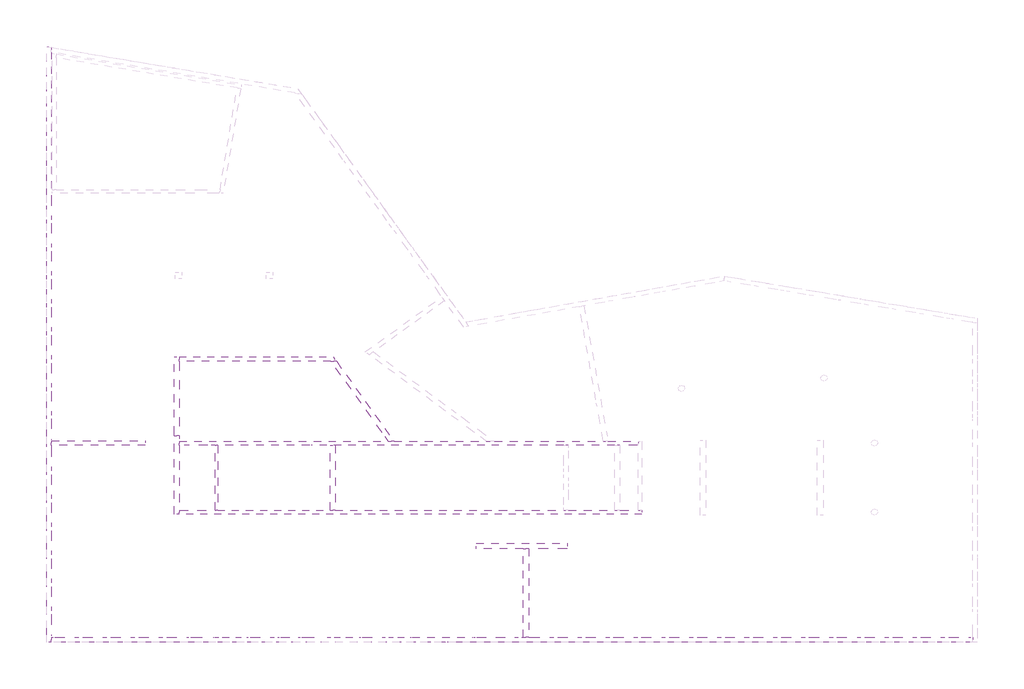
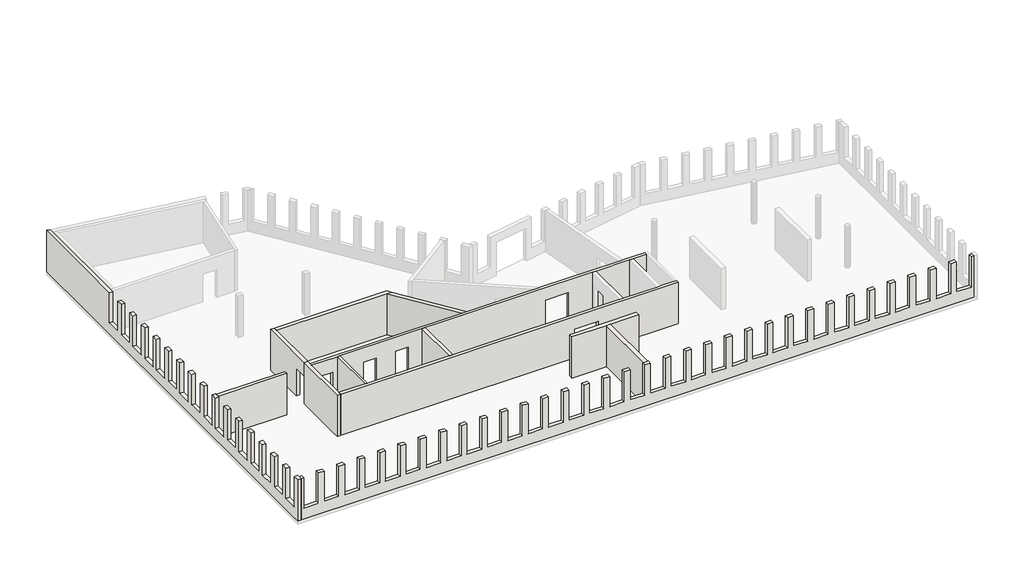
# One storey, part 1 of 2: 13 walls.
# Revit data of these elements (continued)
# Project information (continued)
#   BrowserStrukturXMLData = "<Browserstruktur>\n  <xs:schema id=\"Browserstruktur\" xmlns=\"\" xmlns:xs=\"http://www.w3.org/2001/XMLSchema\" xmlns:msdata=\"urn:schemas-microsoft-com:xml-msdata\">\n    <xs:element name=\"Browserstruktur\" msdata:IsDataSet=\"true\" msdata:MainDataTable=\"ViewTemplates\" msdata:UseCurrentLocale=\"true\">\n      <xs:complexType>\n        <xs:choice minOccurs=\"0\" maxOccurs=\"unbounded\">\n          <xs:element name=\"ViewTemplates\">\n            <xs:complexType>\n              <xs:sequence>\n                <xs:element name=\"Erstellen\" type=\"xs:boolean\" minOccurs=\"0\" />\n                <xs:element name=\"Ansichtsvorlage\" type=\"xs:string\" />\n                <xs:element name=\"_x0031__Fachbereich\" type=\"xs:string\" minOccurs=\"0\" />\n                <xs:element name=\"_x0032__Ansichtstyp\" type=\"xs:string\" minOccurs=\"0\" />\n                <xs:element name=\"_x0033__Ansichtsgruppe\" type=\"xs:string\" minOccurs=\"0\" />\n                <xs:element name=\"Typ\" type=\"xs:string\" minOccurs=\"0\" />\n                <xs:element name=\"Klasse\" type=\"xs:string\" minOccurs=\"0\" />\n                <xs:element name=\"Bedingung\" type=\"xs:string\" minOccurs=\"0\" />\n                <xs:element name=\"Ebenenbezug\" type=\"xs:int\" minOccurs=\"0\" />\n                <xs:element name=\"Ansichtsrichtung\" type=\"xs:string\" minOccurs=\"0\" />\n                <xs:element name=\"Ansichtsname\" type=\"xs:string\" minOccurs=\"0\" />\n              </xs:sequence>\n            </xs:complexType>\n          </xs:element>\n        </xs:choice>\n      </xs:complexType>\n      <xs:unique name=\"Constraint1\" msdata:PrimaryKey=\"true\">\n        <xs:selector xpath=\".//ViewTemplates\" />\n        <xs:field xpath=\"Ansichtsvorlage\" />\n      </xs:unique>\n    </xs:element>\n  </xs:schema>\n  <ViewTemplates>\n    <Erstellen>false</Erstellen>\n    <Ansichtsvorlage>010</Ansichtsvorlage>\n    <_x0031__Fachbereich>00_INTERN</_x0031__Fachbereich>\n    <_x0032__Ansichtstyp>010_CAD_UNTERLAGE</_x0032__Ansichtstyp>\n    <_x0033__Ansichtsgruppe>010_UNTERLAGE_CAD_GESAMT</_x0033__Ansichtsgruppe>\n    <Typ>FloorPlan</Typ>\n    <Klasse>ViewPlan</Klasse>\n    <Bedingung>einmalig</Bedingung>\n    <Ansichtsrichtung>&lt;Ignorieren&gt;</Ansichtsrichtung>\n    <Ansichtsname>[Geschoss_Name]_[Ansichtsgruppe_Name]_[Ebenen_Kommentar]</Ansichtsname>\n  </ViewTemplates>\n  <ViewTemplates>\n    <Erstellen>false</Erstellen>\n    <Ansichtsvorlage>011</Ansichtsvorlage>\n    <_x0031__Fachbereich>00_INTERN</_x0031__Fachbereich>\n    <_x0032__Ansichtstyp>010_CAD_UNTERLAGE</_x0032__Ansichtstyp>\n    <_x0033__Ansichtsgruppe>011_LAGEPLAN</_x0033__Ansichtsgruppe>\n    <Typ>FloorPlan</Typ>\n    <Klasse>ViewPlan</Klasse>\n    <Bedingung>einmalig</Bedingung>\n    <Ansichtsrichtung>&lt;Ignorieren&gt;</Ansichtsrichtung>\n    <Ansichtsname>[Geschoss_Name]_[Ansichtsgruppe_Name]_[Ebenen_Kommentar]</Ansichtsname>\n  </ViewTemplates>\n  <ViewTemplates>\n    <Erstellen>false</Erstellen>\n    <Ansichtsvorlage>025</Ansichtsvorlage>\n    <_x0031__Fachbereich>00_INTERN</_x0031__Fachbereich>\n    <_x0032__Ansichtstyp>010_CAD_UNTERLAGE</_x0032__Ansichtstyp>\n    <_x0033__Ansichtsgruppe>025_ACHSEN</_x0033__Ansichtsgruppe>\n    <Typ>FloorPlan</Typ>\n    <Klasse>ViewPlan</Klasse>\n    <Bedingung>einmalig</Bedingung>\n    <Ansichtsrichtung>&lt;Ignorieren&gt;</Ansichtsrichtung>\n    <Ansichtsname>[Geschoss_Name]_[Ansichtsgruppe_Name]_[Ebenen_Kommentar]</Ansichtsname>\n  </ViewTemplates>\n  <ViewTemplates>\n    <Erstellen>false</Erstellen>\n    <Ansichtsvorlage>030</Ansichtsvorlage>\n    <_x0031__Fachbereich>00_INTERN</_x0031__Fachbereich>\n    <_x0032__Ansichtstyp>010_CAD_UNTERLAGE</_x0032__Ansichtstyp>\n    <_x0033__Ansichtsgruppe>030_ENTWURF_ARCHITEKT</_x0033__Ansichtsgruppe>\n    <Typ>FloorPlan</Typ>\n    <Klasse>ViewPlan</Klasse>\n    <Bedingung>einmalig</Bedingung>\n    <Ebenenbezug>100</Ebenenbezug>\n    <Ansichtsrichtung>&lt;Ignorieren&gt;</Ansichtsrichtung>\n    <Ansichtsname>[Geschoss_Name]_[Ansichtsgruppe_Name]_[Ebenen_Kommentar]</Ansichtsname>\n  </ViewTemplates>\n  <ViewTemplates>\n    <Erstellen>false</Erstellen>\n    <Ansichtsvorlage>060</Ansichtsvorlage>\n    <_x0031__Fachbereich>00_INTERN</_x0031__Fachbereich>\n    <_x0032__Ansichtstyp>060_BILD_UNTERLAGE</_x0032__Ansichtstyp>\n    <_x0033__Ansichtsgruppe>060_UNTERLAGE_BITMAP</_x0033__Ansichtsgruppe>\n    <Typ>FloorPlan</Typ>\n    <Klasse>ViewPlan</Klasse>\n    <Bedingung>einmalig</Bedingung>\n    <Ansichtsrichtung>&lt;Ignorieren&gt;</Ansichtsrichtung>\n    <Ansichtsname>[Geschoss_Name]_[Ansichtsgruppe_Name]_[Ebenen_Kommentar]</Ansichtsname>\n  </ViewTemplates>\n  <ViewTemplates>\n    <Erstellen>false</Erstellen>\n    <Ansichtsvorlage>070</Ansichtsvorlage>\n    <_x0031__Fachbereich>00_INTERN</_x0031__Fachbereich>\n    <_x0032__Ansichtstyp>070_CAD_UEBERLAGE</_x0032__Ansichtstyp>\n    <_x0033__Ansichtsgruppe>070_UEBERLAGE_CAD</_x0033__Ansichtsgruppe>\n    <Typ>FloorPlan</Typ>\n    <Klasse>ViewPlan</Klasse>\n    <Bedingung>einmalig</Bedingung>\n    <Ansichtsrichtung>&lt;Ignorieren&gt;</Ansichtsrichtung>\n    <Ansichtsname>[Geschoss_Name]_[Ansichtsgruppe_Name]_[Ebenen_Kommentar]</Ansichtsname>\n  </ViewTemplates>\n  <ViewTemplates>\n    <Erstellen>false</Erstellen>\n    <Ansichtsvorlage>080</Ansichtsvorlage>\n    <_x0031__Fachbereich>00_INTERN</_x0031__Fachbereich>\n    <_x0032__Ansichtstyp>080_BILD_UEBERLAGE</_x0032__Ansichtstyp>\n    <_x0033__Ansichtsgruppe>080_UEBERLAGE_BITMAP</_x0033__Ansichtsgruppe>\n    <Typ>FloorPlan</Typ>\n    <Klasse>ViewPlan</Klasse>\n    <Bedingung>einmalig</Bedingung>\n    <Ansichtsrichtung>&lt;Ignorieren&gt;</Ansichtsrichtung>\n    <Ansichtsname>[Geschoss_Name]_[Ansichtsgruppe_Name]_[Ebenen_Kommentar]</Ansichtsname>\n  </ViewTemplates>\n  <ViewTemplates>\n    <Erstellen>false</Erstellen>\n    <Ansichtsvorlage>K_5_CC</Ansichtsvorlage>\n    <_x0031__Fachbereich>K_KONSTRUKTION</_x0031__Fachbereich>\n    <_x0032__Ansichtstyp>5_INGENIEUR / ROHBAU</_x0032__Ansichtstyp>\n    <_x0033__Ansichtsgruppe>5_CC_WÄNDE/STÜTZEN</_x0033__Ansichtsgruppe>\n    <Typ>FloorPlan</Typ>\n    <Klasse>ViewPlan</Klasse>\n    <Bedingung>Für jedes Geschoß</Bedingung>\n    <Ebenenbezug>-2</Ebenenbezug>\n    <Ansichtsrichtung>&lt;Ignorieren&gt;</Ansichtsrichtung>\n    <Ansichtsname>[Geschoss_Name]_[Ansichtsgruppe_Name]_[Ebenen_Kommentar]</Ansichtsname>\n  </ViewTemplates>\n  <ViewTemplates>\n    <Erstellen>false</Erstellen>\n    <Ansichtsvorlage>K_5_AA</Ansichtsvorlage>\n    <_x0031__Fachbereich>K_KONSTRUKTION</_x0031__Fachbereich>\n    <_x0032__Ansichtstyp>5_INGENIEUR / ROHBAU</_x0032__Ansichtstyp>\n    <_x0033__Ansichtsgruppe>5_AA_FUNDAMENTE</_x0033__Ansichtsgruppe>\n    <Typ>FloorPlan</Typ>\n    <Klasse>ViewPlan</Klasse>\n    <Bedingung>Für jedes Geschoß</Bedingung>\n    <Ebenenbezug>1000</Ebenenbezug>\n    <Ansichtsrichtung>&lt;Ignorieren&gt;</Ansichtsrichtung>\n    <Ansichtsname>[Geschoss_Name]_[Ansichtsgruppe_Name]_[Ebenen_Kommentar]</Ansichtsname>\n  </ViewTemplates>\n  <ViewTemplates>\n    <Erstellen>false</Erstellen>\n    <Ansichtsvorlage>K_5_BB</Ansichtsvorlage>\n    <_x0031__Fachbereich>K_KONSTRUKTION</_x0031__Fachbereich>\n    <_x0032__Ansichtstyp>5_INGENIEUR / ROHBAU</_x0032__Ansichtstyp>\n    <_x0033__Ansichtsgruppe>5_BB_BODENPLATTE</_x0033__Ansichtsgruppe>\n    <Typ>FloorPlan</Typ>\n    <Klasse>ViewPlan</Klasse>\n    <Bedingung>Für jedes Geschoß</Bedingung>\n    <Ebenenbezug>2</Ebenenbezug>\n    <Ansichtsrichtung>&lt;Ignorieren&gt;</Ansichtsrichtung>\n    <Ansichtsname>[Geschoss_Name]_[Ansichtsgruppe_Name]_[Ebenen_Kommentar]</Ansichtsname>\n  </ViewTemplates>\n  <ViewTemplates>\n    <Erstellen>false</Erstellen>\n    <Ansichtsvorlage>K_5_EE</Ansichtsvorlage>\n    <_x0031__Fachbereich>K_KONSTRUKTION</_x0031__Fachbereich>\n    <_x0032__Ansichtstyp>5_INGENIEUR / ROHBAU</_x0032__Ansichtstyp>\n    <_x0033__Ansichtsgruppe>5_EE_GESCHOSSDECKEN</_x0033__Ansichtsgruppe>\n    <Typ>FloorPlan</Typ>\n    <Klasse>ViewPlan</Klasse>\n    <Bedingung>Für jedes Geschoß</Bedingung>\n    <Ebenenbezug>2</Ebenenbezug>\n    <Ansichtsrichtung>&lt;Ignorieren&gt;</Ansichtsrichtung>\n    <Ansichtsname>[Geschoss_Name]_[Ansichtsgruppe_Name]_[Ebenen_Kommentar]</Ansichtsname>\n  </ViewTemplates>\n  <ViewTemplates>\n    <Erstellen>false</Erstellen>\n    <Ansichtsvorlage>K_6b_AA</Ansichtsvorlage>\n    <_x0031__Fachbereich>K_KONSTRUKTION</_x0031__Fachbereich>\n    <_x0032__Ansichtstyp>6b_FASSADE</_x0032__Ansichtstyp>\n    <_x0033__Ansichtsgruppe>6b_AA_FENSTER_UND_GLASFASSADE</_x0033__Ansichtsgruppe>\n    <Typ>FloorPlan</Typ>\n    <Klasse>ViewPlan</Klasse>\n    <Bedingung>Für jedes Geschoß</Bedingung>\n    <Ebenenbezug>-2</Ebenenbezug>\n    <Ansichtsrichtung>&lt;Ignorieren&gt;</Ansichtsrichtung>\n    <Ansichtsname>[Geschoss_Name]_[Ansichtsgruppe_Name]_[Ebenen_Kommentar]</Ansichtsname>\n  </ViewTemplates>\n  <ViewTemplates>\n    <Erstellen>false</Erstellen>\n    <Ansichtsvorlage>K_6b_DD</Ansichtsvorlage>\n    <_x0031__Fachbereich>K_KONSTRUKTION</_x0031__Fachbereich>\n    <_x0032__Ansichtstyp>6b_FASSADE</_x0032__Ansichtstyp>\n    <_x0033__Ansichtsgruppe>6b_DD_AUßENPUTZ_WDVS</_x0033__Ansichtsgruppe>\n    <Typ>FloorPlan</Typ>\n    <Klasse>ViewPlan</Klasse>\n    <Bedingung>Für jedes Geschoß</Bedingung>\n    <Ebenenbezug>-2</Ebenenbezug>\n    <Ansichtsrichtung>&lt;Ignorieren&gt;</Ansichtsrichtung>\n    <Ansichtsname>[Geschoss_Name]_[Ansichtsgruppe_Name]_[Ebenen_Kommentar]</Ansichtsname>\n  </ViewTemplates>\n  <ViewTemplates>\n    <Erstellen>false</Erstellen>\n    <Ansichtsvorlage>K_5_S1_AA</Ansichtsvorlage>\n    <_x0031__Fachbereich>K_KONSTRUKTION</_x0031__Fachbereich>\n    <_x0032__Ansichtstyp>5_S1_STATIK</_x0032__Ansichtstyp>\n    <_x0033__Ansichtsgruppe>5_S1_AA_GRUNDRISSE</_x0033__Ansichtsgruppe>\n    <Typ>FloorPlan</Typ>\n    <Klasse>ViewPlan</Klasse>\n    <Bedingung>Für jedes Geschoß</Bedingung>\n    <Ebenenbezug>-2</Ebenenbezug>\n    <Ansichtsrichtung>&lt;Ignorieren&gt;</Ansichtsrichtung>\n    <Ansichtsname>[Geschoss_Name]_[Ansichtsgruppe_Name]_[Ebenen_Kommentar]</Ansichtsname>\n  </ViewTemplates>\n  <ViewTemplates>\n    <Erstellen>false</Erstellen>\n    <Ansichtsvorlage>K_5_S2_AA</Ansichtsvorlage>\n    <_x0031__Fachbereich>K_KONSTRUKTION</_x0031__Fachbereich>\n    <_x0032__Ansichtstyp>5_S2_BEWEHRUNG</_x0032__Ansichtstyp>\n    <_x0033__Ansichtsgruppe>5_S2_AA_GRUNDRISSE</_x0033__Ansichtsgruppe>\n    <Typ>FloorPlan</Typ>\n    <Klasse>ViewPlan</Klasse>\n    <Bedingung>Für jedes Geschoß</Bedingung>\n    <Ebenenbezug>-2</Ebenenbezug>\n    <Ansichtsrichtung>&lt;Ignorieren&gt;</Ansichtsrichtung>\n    <Ansichtsname>[Geschoss_Name]_[Ansichtsgruppe_Name]_[Ebenen_Kommentar]</Ansichtsname>\n  </ViewTemplates>\n  <ViewTemplates>\n    <Erstellen>false</Erstellen>\n    <Ansichtsvorlage>K_5_DD</Ansichtsvorlage>\n    <_x0031__Fachbereich>K_KONSTRUKTION</_x0031__Fachbereich>\n    <_x0032__Ansichtstyp>5_INGENIEUR / ROHBAU</_x0032__Ansichtstyp>\n    <_x0033__Ansichtsgruppe>5_DD_TRÄGER</_x0033__Ansichtsgruppe>\n    <Typ>FloorPlan</Typ>\n    <Klasse>ViewPlan</Klasse>\n    <Bedingung>Für jedes Geschoß</Bedingung>\n    <Ebenenbezug>1</Ebenenbezug>\n    <Ansichtsrichtung>&lt;Ignorieren&gt;</Ansichtsrichtung>\n    <Ansichtsname>[Geschoss_Name]_[Ansichtsgruppe_Name]_[Ebenen_Kommentar]</Ansichtsname>\n  </ViewTemplates>\n  <ViewTemplates>\n    <Erstellen>false</Erstellen>\n    <Ansichtsvorlage>K_5_S1_BB</Ansichtsvorlage>\n    <_x0031__Fachbereich>K_KONSTRUKTION</_x0031__Fachbereich>\n    <_x0032__Ansichtstyp>5_S1_STATIK</_x0032__Ansichtstyp>\n    <_x0033__Ansichtsgruppe>5_S1_BB_DECKENSPIEGEL</_x0033__Ansichtsgruppe>\n    <Typ>FloorPlan</Typ>\n    <Klasse>ViewPlan</Klasse>\n    <Bedingung>Für jedes Geschoß</Bedingung>\n    <Ebenenbezug>2</Ebenenbezug>\n    <Ansichtsrichtung>&lt;Ignorieren&gt;</Ansichtsrichtung>\n    <Ansichtsname>[Geschoss_Name]_[Ansichtsgruppe_Name]_[Ebenen_Kommentar]</Ansichtsname>\n  </ViewTemplates>\n  <ViewTemplates>\n    <Erstellen>false</Erstellen>\n    <Ansichtsvor
#     lage>K_5_S2_BB</Ansichtsvorlage>\n    <_x0031__Fachbereich>K_KONSTRUKTION</_x0031__Fachbereich>\n    <_x0032__Ansichtstyp>5_S2_BEWEHRUNG</_x0032__Ansichtstyp>\n    <_x0033__Ansichtsgruppe>5_S2_BB_DECKENSPIEGEL</_x0033__Ansichtsgruppe>\n    <Typ>FloorPlan</Typ>\n    <Klasse>ViewPlan</Klasse>\n    <Bedingung>Für jedes Geschoß</Bedingung>\n    <Ebenenbezug>2</Ebenenbezug>\n    <Ansichtsrichtung>&lt;Ignorieren&gt;</Ansichtsrichtung>\n    <Ansichtsname>[Geschoss_Name]_[Ansichtsgruppe_Name]_[Ebenen_Kommentar]</Ansichtsname>\n  </ViewTemplates>\n  <ViewTemplates>\n    <Erstellen>false</Erstellen>\n    <Ansichtsvorlage>K_6b_BB</Ansichtsvorlage>\n    <_x0031__Fachbereich>K_KONSTRUKTION</_x0031__Fachbereich>\n    <_x0032__Ansichtstyp>6b_FASSADE</_x0032__Ansichtstyp>\n    <_x0033__Ansichtsgruppe>6b_BB_FASSADENBEKLEIDUNG</_x0033__Ansichtsgruppe>\n    <Typ>FloorPlan</Typ>\n    <Klasse>ViewPlan</Klasse>\n    <Bedingung>Für jedes Geschoß</Bedingung>\n    <Ebenenbezug>2</Ebenenbezug>\n    <Ansichtsrichtung>&lt;Ignorieren&gt;</Ansichtsrichtung>\n    <Ansichtsname>[Geschoss_Name]_[Ansichtsgruppe_Name]_[Ebenen_Kommentar]</Ansichtsname>\n  </ViewTemplates>\n  <ViewTemplates>\n    <Erstellen>false</Erstellen>\n    <Ansichtsvorlage>K_6b_CC</Ansichtsvorlage>\n    <_x0031__Fachbereich>K_KONSTRUKTION</_x0031__Fachbereich>\n    <_x0032__Ansichtstyp>6b_FASSADE</_x0032__Ansichtstyp>\n    <_x0033__Ansichtsgruppe>6b_CC_SONNENSCHUTZ_BLENDSCHUTZ</_x0033__Ansichtsgruppe>\n    <Typ>FloorPlan</Typ>\n    <Klasse>ViewPlan</Klasse>\n    <Bedingung>Für jedes Geschoß</Bedingung>\n    <Ebenenbezug>2</Ebenenbezug>\n    <Ansichtsrichtung>&lt;Ignorieren&gt;</Ansichtsrichtung>\n    <Ansichtsname>[Geschoss_Name]_[Ansichtsgruppe_Name]_[Ebenen_Kommentar]</Ansichtsname>\n  </ViewTemplates>\n  <ViewTemplates>\n    <Erstellen>false</Erstellen>\n    <Ansichtsvorlage>K_6c_AA</Ansichtsvorlage>\n    <_x0031__Fachbereich>K_KONSTRUKTION</_x0031__Fachbereich>\n    <_x0032__Ansichtstyp>6c_AUSBAU</_x0032__Ansichtstyp>\n    <_x0033__Ansichtsgruppe>6c_AA_WÄNDE_ALLGEMEIN</_x0033__Ansichtsgruppe>\n    <Typ>FloorPlan</Typ>\n    <Klasse>ViewPlan</Klasse>\n    <Bedingung>Für jedes Geschoß</Bedingung>\n    <Ebenenbezug>-2</Ebenenbezug>\n    <Ansichtsrichtung>&lt;Ignorieren&gt;</Ansichtsrichtung>\n    <Ansichtsname>[Geschoss_Name]_[Ansichtsgruppe_Name]_[Ebenen_Kommentar]</Ansichtsname>\n  </ViewTemplates>\n  <ViewTemplates>\n    <Erstellen>false</Erstellen>\n    <Ansichtsvorlage>K_6c_AC</Ansichtsvorlage>\n    <_x0031__Fachbereich>K_KONSTRUKTION</_x0031__Fachbereich>\n    <_x0032__Ansichtstyp>6c_AUSBAU</_x0032__Ansichtstyp>\n    <_x0033__Ansichtsgruppe>6c_AC_SYSTEMTRENNWÄNDE</_x0033__Ansichtsgruppe>\n    <Typ>FloorPlan</Typ>\n    <Klasse>ViewPlan</Klasse>\n    <Bedingung>Für jedes Geschoß</Bedingung>\n    <Ebenenbezug>3</Ebenenbezug>\n    <Ansichtsrichtung>&lt;Ignorieren&gt;</Ansichtsrichtung>\n    <Ansichtsname>[Geschoss_Name]_[Ansichtsgruppe_Name]_[Ebenen_Kommentar]</Ansichtsname>\n  </ViewTemplates>\n  <ViewTemplates>\n    <Erstellen>false</Erstellen>\n    <Ansichtsvorlage>K_6c_BX</Ansichtsvorlage>\n    <_x0031__Fachbereich>K_KONSTRUKTION</_x0031__Fachbereich>\n    <_x0032__Ansichtstyp>6c_AUSBAU</_x0032__Ansichtstyp>\n    <_x0033__Ansichtsgruppe>6c_BX_RÄUME (RAUMBEZEICHNUNGEN)</_x0033__Ansichtsgruppe>\n    <Typ>FloorPlan</Typ>\n    <Klasse>ViewPlan</Klasse>\n    <Bedingung>Für jedes Geschoß</Bedingung>\n    <Ebenenbezug>3</Ebenenbezug>\n    <Ansichtsrichtung>&lt;Ignorieren&gt;</Ansichtsrichtung>\n    <Ansichtsname>[Geschoss_Name]_[Ansichtsgruppe_Name]_[Ebenen_Kommentar]</Ansichtsname>\n  </ViewTemplates>\n  <ViewTemplates>\n    <Erstellen>false</Erstellen>\n    <Ansichtsvorlage>K_6c_BY</Ansichtsvorlage>\n    <_x0031__Fachbereich>K_KONSTRUKTION</_x0031__Fachbereich>\n    <_x0032__Ansichtstyp>6c_AUSBAU</_x0032__Ansichtstyp>\n    <_x0033__Ansichtsgruppe>6c_BY_RÄUME (NUTZFLÄCHEN NACH DIN 277)</_x0033__Ansichtsgruppe>\n    <Typ>FloorPlan</Typ>\n    <Klasse>ViewPlan</Klasse>\n    <Bedingung>Für jedes Geschoß</Bedingung>\n    <Ebenenbezug>3</Ebenenbezug>\n    <Ansichtsrichtung>&lt;Ignorieren&gt;</Ansichtsrichtung>\n    <Ansichtsname>[Geschoss_Name]_[Ansichtsgruppe_Name]_[Ebenen_Kommentar]</Ansichtsname>\n  </ViewTemplates>\n  <ViewTemplates>\n    <Erstellen>false</Erstellen>\n    <Ansichtsvorlage>K_6c_CA</Ansichtsvorlage>\n    <_x0031__Fachbereich>K_KONSTRUKTION</_x0031__Fachbereich>\n    <_x0032__Ansichtstyp>6c_AUSBAU</_x0032__Ansichtstyp>\n    <_x0033__Ansichtsgruppe>6c_CA_TÜREN_ALLGEMEIN</_x0033__Ansichtsgruppe>\n    <Typ>FloorPlan</Typ>\n    <Klasse>ViewPlan</Klasse>\n    <Bedingung>Für jedes Geschoß</Bedingung>\n    <Ebenenbezug>-2</Ebenenbezug>\n    <Ansichtsrichtung>&lt;Ignorieren&gt;</Ansichtsrichtung>\n    <Ansichtsname>[Geschoss_Name]_[Ansichtsgruppe_Name]_[Ebenen_Kommentar]</Ansichtsname>\n  </ViewTemplates>\n  <ViewTemplates>\n    <Erstellen>false</Erstellen>\n    <Ansichtsvorlage>K_6c_CB</Ansichtsvorlage>\n    <_x0031__Fachbereich>K_KONSTRUKTION</_x0031__Fachbereich>\n    <_x0032__Ansichtstyp>6c_AUSBAU</_x0032__Ansichtstyp>\n    <_x0033__Ansichtsgruppe>6c_CB_HOLZTÜREN (TYPEN)</_x0033__Ansichtsgruppe>\n    <Typ>FloorPlan</Typ>\n    <Klasse>ViewPlan</Klasse>\n    <Bedingung>Für jedes Geschoß</Bedingung>\n    <Ebenenbezug>-2</Ebenenbezug>\n    <Ansichtsrichtung>&lt;Ignorieren&gt;</Ansichtsrichtung>\n    <Ansichtsname>[Geschoss_Name]_[Ansichtsgruppe_Name]_[Ebenen_Kommentar]</Ansichtsname>\n  </ViewTemplates>\n  <ViewTemplates>\n    <Erstellen>false</Erstellen>\n    <Ansichtsvorlage>K_6c_CC</Ansichtsvorlage>\n    <_x0031__Fachbereich>K_KONSTRUKTION</_x0031__Fachbereich>\n    <_x0032__Ansichtstyp>6c_AUSBAU</_x0032__Ansichtstyp>\n    <_x0033__Ansichtsgruppe>6c_CC_BLECHTÜREN (TYPEN)</_x0033__Ansichtsgruppe>\n    <Typ>FloorPlan</Typ>\n    <Klasse>ViewPlan</Klasse>\n    <Bedingung>Für jedes Geschoß</Bedingung>\n    <Ebenenbezug>-2</Ebenenbezug>\n    <Ansichtsrichtung>&lt;Ignorieren&gt;</Ansichtsrichtung>\n    <Ansichtsname>[Geschoss_Name]_[Ansichtsgruppe_Name]_[Ebenen_Kommentar]</Ansichtsname>\n  </ViewTemplates>\n  <ViewTemplates>\n    <Erstellen>false</Erstellen>\n    <Ansichtsvorlage>K_6c_CD</Ansichtsvorlage>\n    <_x0031__Fachbereich>K_KONSTRUKTION</_x0031__Fachbereich>\n    <_x0032__Ansichtstyp>6c_AUSBAU</_x0032__Ansichtstyp>\n    <_x0033__Ansichtsgruppe>6c_CD_ROHRRAHMENTÜREN (TYPEN)</_x0033__Ansichtsgruppe>\n    <Typ>FloorPlan</Typ>\n    <Klasse>ViewPlan</Klasse>\n    <Bedingung>Für jedes Geschoß</Bedingung>\n    <Ebenenbezug>-2</Ebenenbezug>\n    <Ansichtsrichtung>&lt;Ignorieren&gt;</Ansichtsrichtung>\n    <Ansichtsname>[Geschoss_Name]_[Ansichtsgruppe_Name]_[Ebenen_Kommentar]</Ansichtsname>\n  </ViewTemplates>\n  <ViewTemplates>\n    <Erstellen>false</Erstellen>\n    <Ansichtsvorlage>K_6c_CE</Ansichtsvorlage>\n    <_x0031__Fachbereich>K_KONSTRUKTION</_x0031__Fachbereich>\n    <_x0032__Ansichtstyp>6c_AUSBAU</_x0032__Ansichtstyp>\n    <_x0033__Ansichtsgruppe>6c_CE_SPEZIALTÜREN/TORE</_x0033__Ansichtsgruppe>\n    <Typ>FloorPlan</Typ>\n    <Klasse>ViewPlan</Klasse>\n    <Bedingung>Für jedes Geschoß</Bedingung>\n    <Ebenenbezug>-2</Ebenenbezug>\n    <Ansichtsrichtung>&lt;Ignorieren&gt;</Ansichtsrichtung>\n    <Ansichtsname>[Geschoss_Name]_[Ansichtsgruppe_Name]_[Ebenen_Kommentar]</Ansichtsname>\n  </ViewTemplates>\n  <ViewTemplates>\n    <Erstellen>false</Erstellen>\n    <Ansichtsvorlage>K_6c_DA</Ansichtsvorlage>\n    <_x0031__Fachbereich>K_KONSTRUKTION</_x0031__Fachbereich>\n    <_x0032__Ansichtstyp>6c_AUSBAU</_x0032__Ansichtstyp>\n    <_x0033__Ansichtsgruppe>6c_DA_BODENKONSTRUKTION (TYPEN)</_x0033__Ansichtsgruppe>\n    <Typ>FloorPlan</Typ>\n    <Klasse>ViewPlan</Klasse>\n    <Bedingung>Für jedes Geschoß</Bedingung>\n    <Ebenenbezug>3</Ebenenbezug>\n    <Ansichtsrichtung>&lt;Ignorieren&gt;</Ansichtsrichtung>\n    <Ansichtsname>[Geschoss_Name]_[Ansichtsgruppe_Name]_[Ebenen_Kommentar]</Ansichtsname>\n  </ViewTemplates>\n  <ViewTemplates>\n    <Erstellen>false</Erstellen>\n    <Ansichtsvorlage>K_6c_AD</Ansichtsvorlage>\n    <_x0031__Fachbereich>K_KONSTRUKTION</_x0031__Fachbereich>\n    <_x0032__Ansichtstyp>6c_AUSBAU</_x0032__Ansichtstyp>\n    <_x0033__Ansichtsgruppe>6c_AD_WC_TRENNWÄNDE</_x0033__Ansichtsgruppe>\n    <Typ>FloorPlan</Typ>\n    <Klasse>ViewPlan</Klasse>\n    <Bedingung>Für jedes Geschoß</Bedingung>\n    <Ebenenbezug>3</Ebenenbezug>\n    <Ansichtsrichtung>&lt;Ignorieren&gt;</Ansichtsrichtung>\n    <Ansichtsname>[Geschoss_Name]_[Ansichtsgruppe_Name]_[Ebenen_Kommentar]</Ansichtsname>\n  </ViewTemplates>\n  <ViewTemplates>\n    <Erstellen>false</Erstellen>\n    <Ansichtsvorlage>K_5_FF</Ansichtsvorlage>\n    <_x0031__Fachbereich>K_KONSTRUKTION</_x0031__Fachbereich>\n    <_x0032__Ansichtstyp>5_INGENIEUR / ROHBAU</_x0032__Ansichtstyp>\n    <_x0033__Ansichtsgruppe>5_FF_EINBAUTEILE</_x0033__Ansichtsgruppe>\n    <Typ>FloorPlan</Typ>\n    <Klasse>ViewPlan</Klasse>\n    <Bedingung>Auswahl</Bedingung>\n    <Ebenenbezug>2</Ebenenbezug>\n    <Ansichtsrichtung>&lt;Ignorieren&gt;</Ansichtsrichtung>\n    <Ansichtsname>[Geschoss_Name]_[Ansichtsgruppe_Name]_[Ebenen_Kommentar]</Ansichtsname>\n  </ViewTemplates>\n  <ViewTemplates>\n    <Erstellen>false</Erstellen>\n    <Ansichtsvorlage>K_5_GG</Ansichtsvorlage>\n    <_x0031__Fachbereich>K_KONSTRUKTION</_x0031__Fachbereich>\n    <_x0032__Ansichtstyp>5_INGENIEUR / ROHBAU</_x0032__Ansichtstyp>\n    <_x0033__Ansichtsgruppe>5_GG_SONSTIGE_BAUTEILE</_x0033__Ansichtsgruppe>\n    <Typ>FloorPlan</Typ>\n    <Klasse>ViewPlan</Klasse>\n    <Bedingung>Auswahl</Bedingung>\n    <Ebenenbezug>2</Ebenenbezug>\n    <Ansichtsrichtung>&lt;Ignorieren&gt;</Ansichtsrichtung>\n    <Ansichtsname>[Geschoss_Name]_[Ansichtsgruppe_Name]_[Ebenen_Kommentar]</Ansichtsname>\n  </ViewTemplates>\n  <ViewTemplates>\n    <Erstellen>false</Erstellen>\n    <Ansichtsvorlage>K_6c_AE</Ansichtsvorlage>\n    <_x0031__Fachbereich>K_KONSTRUKTION</_x0031__Fachbereich>\n    <_x0032__Ansichtstyp>6c_AUSBAU</_x0032__Ansichtstyp>\n    <_x0033__Ansichtsgruppe>6c_AE_KELLER</_x0033__Ansichtsgruppe>\n    <Typ>FloorPlan</Typ>\n    <Klasse>ViewPlan</Klasse>\n    <Bedingung>Für jedes Geschoß</Bedingung>\n    <Ebenenbezug>3</Ebenenbezug>\n    <Ansichtsrichtung>&lt;Ignorieren&gt;</Ansichtsrichtung>\n    <Ansichtsname>[Geschoss_Name]_[Ansichtsgruppe_Name]_[Ebenen_Kommentar]</Ansichtsname>\n  </ViewTemplates>\n  <ViewTemplates>\n    <Erstellen>false</Erstellen>\n    <Ansichtsvorlage>K_6c_BA</Ansichtsvorlage>\n    <_x0031__Fachbereich>K_KONSTRUKTION</_x0031__Fachbereich>\n    <_x0032__Ansichtstyp>6c_AUSBAU</_x0032__Ansichtstyp>\n    <_x0033__Ansichtsgruppe>6c_BA_RÄUME (TYPEN)</_x0033__Ansichtsgruppe>\n    <Typ>FloorPlan</Typ>\n    <Klasse>ViewPlan</Klasse>\n    <Bedingung>Für jedes Geschoß</Bedingung>\n    <Ebenenbezug>3</Ebenenbezug>\n    <Ansichtsrichtung>&lt;Ignorieren&gt;</Ansichtsrichtung>\n    <Ansichtsname>[Geschoss_Name]_[Ansichtsgruppe_Name]_[Ebenen_Kommentar]</Ansichtsname>\n  </ViewTemplates>\n  <ViewTemplates>\n    <Erstellen>false</Erstellen>\n    <Ansichtsvorlage>K_6c_BB</Ansichtsvorlage>\n    <_x0031__Fachbereich>K_KONSTRUKTION</_x0031__Fachbereich>\n    <_x0032__Ansichtstyp>6c_AUSBAU</_x0032__Ansichtstyp>\n    <_x0033__Ansichtsgruppe>6c_BB_RAUM_SPEZIAL_OBERFLÄCHEN</_x0033__Ansichtsgruppe>\n    <Typ>FloorPlan</Typ>\n    <Klasse>ViewPlan</Klasse>\n    <Bedingung>Für jedes Geschoß</Bedingung>\n    <Ebenenbezug>3</Ebenenbezug>\n    <Ansichtsrichtung>&lt;Ignorieren&gt;</Ansichtsrichtung>\n    <Ansichtsname>[Geschoss_Name]_[Ansichtsgruppe_Name]_[Ebenen_Kommentar]</Ansichtsname>\n  </ViewTemplates>\n  <ViewTemplates>\n    <Erstellen>false</Erstellen>\n    <Ansichtsvorlage>K_6c_AB</Ansichtsvorlage>\n    <_x0031__Fachbereich>K_KONSTRUKTION</_x0031__Fachbereich>\n    <_x0032__Ansichtstyp>6c_AUSBAU</_x0032__Ansichtstyp>\n    <_x0033__Ansichtsgruppe>6c_AB_GK_WÄNDE</_x0033__Ansichtsgruppe>\n    <Typ>FloorPlan</Typ>\n    <Klasse>ViewPlan</Klasse>\n    <Bedingung>Für jedes Geschoß</Bedingung>\n    <Ebenenbezug>-2</Ebenenbezug>\n    <Ansichtsrichtung>&lt;Ignoriere
#     n&gt;</Ansichtsrichtung>\n    <Ansichtsname>[Geschoss_Name]_[Ansichtsgruppe_Name]_[Ebenen_Kommentar]</Ansichtsname>\n  </ViewTemplates>\n  <ViewTemplates>\n    <Erstellen>false</Erstellen>\n    <Ansichtsvorlage>K_6c_EA</Ansichtsvorlage>\n    <_x0031__Fachbereich>K_KONSTRUKTION</_x0031__Fachbereich>\n    <_x0032__Ansichtstyp>6c_AUSBAU</_x0032__Ansichtstyp>\n    <_x0033__Ansichtsgruppe>6c_EA_ABGEHÄNGTE_DECKEN (TYPEN)</_x0033__Ansichtsgruppe>\n    <Typ>CeilingPlan</Typ>\n    <Klasse>ViewPlan</Klasse>\n    <Bedingung>Für jedes Geschoß</Bedingung>\n    <Ebenenbezug>4</Ebenenbezug>\n    <Ansichtsrichtung>&lt;Ignorieren&gt;</Ansichtsrichtung>\n    <Ansichtsname>[Geschoss_Name]_[Ansichtsgruppe_Name]_[Ebenen_Kommentar]</Ansichtsname>\n  </ViewTemplates>\n  <ViewTemplates>\n    <Erstellen>true</Erstellen>\n    <Ansichtsvorlage>P_5_P2_NEU</Ansichtsvorlage>\n    <_x0031__Fachbereich>P_PLANBEREICH</_x0031__Fachbereich>\n    <_x0032__Ansichtstyp>5_INGENIEUR / ROHBAU</_x0032__Ansichtstyp>\n    <_x0033__Ansichtsgruppe>5_P2_SCHALPLÄNE</_x0033__Ansichtsgruppe>\n    <Typ>CeilingPlan</Typ>\n    <Klasse>ViewPlan</Klasse>\n    <Bedingung>Für jedes Geschoß</Bedingung>\n    <Ebenenbezug>-2</Ebenenbezug>\n    <Ansichtsrichtung>&lt;Ignorieren&gt;</Ansichtsrichtung>\n    <Ansichtsname>[Geschoss_Name]_[Ansichtsgruppe_Name]_[Ebenen_Kommentar]</Ansichtsname>\n  </ViewTemplates>\n  <ViewTemplates>\n    <Erstellen>false</Erstellen>\n    <Ansichtsvorlage>P_5_P3</Ansichtsvorlage>\n    <_x0031__Fachbereich>P_PLANBEREICH</_x0031__Fachbereich>\n    <_x0032__Ansichtstyp>5_INGENIEUR / ROHBAU</_x0032__Ansichtstyp>\n    <_x0033__Ansichtsgruppe>5_P3_BEWEHRUNGSPLÄNE</_x0033__Ansichtsgruppe>\n    <Typ>CeilingPlan</Typ>\n    <Klasse>ViewPlan</Klasse>\n    <Bedingung>Für jedes Geschoß</Bedingung>\n    <Ebenenbezug>-2</Ebenenbezug>\n    <Ansichtsrichtung>&lt;Ignorieren&gt;</Ansichtsrichtung>\n    <Ansichtsname>[Geschoss_Name]_[Ansichtsgruppe_Name]_[Ebenen_Kommentar]</Ansichtsname>\n  </ViewTemplates>\n  <ViewTemplates>\n    <Erstellen>true</Erstellen>\n    <Ansichtsvorlage>P_5_P2_AW_NEU</Ansichtsvorlage>\n    <_x0031__Fachbereich>P_PLANBEREICH</_x0031__Fachbereich>\n    <_x0032__Ansichtstyp>5_INGENIEUR / ROHBAU</_x0032__Ansichtstyp>\n    <_x0033__Ansichtsgruppe>5_P2_SCHALPLÄNE_VK</_x0033__Ansichtsgruppe>\n    <Typ>CeilingPlan</Typ>\n    <Klasse>ViewPlan</Klasse>\n    <Bedingung>Für jedes Geschoß</Bedingung>\n    <Ebenenbezug>2</Ebenenbezug>\n    <Ansichtsrichtung>&lt;Ignorieren&gt;</Ansichtsrichtung>\n    <Ansichtsname>[Geschoss_Name]_[Ansichtsgruppe_Name]_[Ebenen_Kommentar]</Ansichtsname>\n  </ViewTemplates>\n  <ViewTemplates>\n    <Ansichtsvorlage>P_5_CC_NEU</Ansichtsvorlage>\n    <_x0031__Fachbereich>P_PLANBEREICH</_x0031__Fachbereich>\n    <_x0032__Ansichtstyp>5_INGENIEUR / ROHBAU</_x0032__Ansichtstyp>\n    <_x0033__Ansichtsgruppe>5_CC_WÄNDE/STÜTZEN</_x0033__Ansichtsgruppe>\n    <Typ>FloorPlan</Typ>\n    <Klasse>ViewPlan</Klasse>\n    <Bedingung>Für jedes Geschoß</Bedingung>\n    <Ebenenbezug>-2</Ebenenbezug>\n    <Ansichtsrichtung>&lt;Ignorieren&gt;</Ansichtsrichtung>\n    <Ansichtsname>[Geschoss_Name]_[Ansichtsgruppe_Name]_[Ebenen_Kommentar]</Ansichtsname>\n  </ViewTemplates>\n</Browserstruktur>"
#   PrintManagerSettings = "<PrintManagerDS xmlns=\"http://tempuri.org/PrintManagerDS.xsd\">\n  <xs:schema id=\"PrintManagerDS\" targetNamespace=\"http://tempuri.org/PrintManagerDS.xsd\" xmlns:mstns=\"http://tempuri.org/PrintManagerDS.xsd\" xmlns=\"http://tempuri.org/PrintManagerDS.xsd\" xmlns:xs=\"http://www.w3.org/2001/XMLSchema\" xmlns:msdata=\"urn:schemas-microsoft-com:xml-msdata\" attributeFormDefault=\"qualified\" elementFormDefault=\"qualified\">\n    <xs:element name=\"PrintManagerDS\" msdata:IsDataSet=\"true\" msdata:UseCurrentLocale=\"true\">\n      <xs:complexType>\n        <xs:choice minOccurs=\"0\" maxOccurs=\"unbounded\">\n          <xs:element name=\"DruckEinstellungDT\">\n            <xs:complexType>\n              <xs:sequence>\n                <xs:element name=\"ID\" msdata:DataType=\"System.Guid, mscorlib, Version=4.0.0.0, Culture=neutral, PublicKeyToken=b77a5c561934e089\" msdata:AutoIncrementSeed=\"-1\" msdata:AutoIncrementStep=\"-1\" type=\"xs:string\" minOccurs=\"0\" />\n                <xs:element name=\"Name\" type=\"xs:string\" minOccurs=\"0\" />\n                <xs:element name=\"Beschreibung\" type=\"xs:string\" minOccurs=\"0\" />\n                <xs:element name=\"Kategorie\" type=\"xs:string\" minOccurs=\"0\" />\n                <xs:element name=\"PrinterName\" type=\"xs:string\" minOccurs=\"0\" />\n                <xs:element name=\"PrintToFile\" type=\"xs:boolean\" minOccurs=\"0\" />\n                <xs:element name=\"FileName\" type=\"xs:string\" minOccurs=\"0\" />\n                <xs:element name=\"ColorDepth\" type=\"xs:string\" minOccurs=\"0\" />\n                <xs:element name=\"HiddenLineViews\" type=\"xs:string\" minOccurs=\"0\" />\n                <xs:element name=\"HideCropBoundaries\" type=\"xs:boolean\" minOccurs=\"0\" />\n                <xs:element name=\"HideRefOrWorkPlanes\" type=\"xs:boolean\" minOccurs=\"0\" />\n                <xs:element name=\"HideScopeBoxes\" type=\"xs:boolean\" minOccurs=\"0\" />\n                <xs:element name=\"HideUnreferencedViewTags\" type=\"xs:boolean\" minOccurs=\"0\" />\n                <xs:element name=\"MarginType\" type=\"xs:string\" minOccurs=\"0\" />\n                <xs:element name=\"PageOrientation\" type=\"xs:string\" minOccurs=\"0\" />\n                <xs:element name=\"PaperPlacement\" type=\"xs:string\" minOccurs=\"0\" />\n                <xs:element name=\"PaperSize\" type=\"xs:string\" minOccurs=\"0\" />\n                <xs:element name=\"PaperSource\" type=\"xs:string\" minOccurs=\"0\" />\n                <xs:element name=\"RasterQuality\" type=\"xs:string\" minOccurs=\"0\" />\n                <xs:element name=\"ReplaceHalftoneWithThinLines\" type=\"xs:boolean\" minOccurs=\"0\" />\n                <xs:element name=\"UserDefinedMarginX\" type=\"xs:double\" minOccurs=\"0\" />\n                <xs:element name=\"UserDefinedMarginY\" type=\"xs:double\" minOccurs=\"0\" />\n                <xs:element name=\"ViewLinksInBlue\" type=\"xs:boolean\" minOccurs=\"0\" />\n                <xs:element name=\"Zoom\" type=\"xs:int\" minOccurs=\"0\" />\n                <xs:element name=\"ZoomType\" type=\"xs:string\" minOccurs=\"0\" />\n              </xs:sequence>\n            </xs:complexType>\n          </xs:element>\n          <xs:element name=\"DruckSatzDT\">\n            <xs:complexType>\n              <xs:sequence>\n                <xs:element name=\"ID\" msdata:DataType=\"System.Guid, mscorlib, Version=4.0.0.0, Culture=neutral, PublicKeyToken=b77a5c561934e089\" type=\"xs:string\" minOccurs=\"0\" />\n                <xs:element name=\"PlanID\" type=\"xs:string\" minOccurs=\"0\" />\n                <xs:element name=\"DruckEinstellungID\" msdata:DataType=\"System.Guid, mscorlib, Version=4.0.0.0, Culture=neutral, PublicKeyToken=b77a5c561934e089\" type=\"xs:string\" minOccurs=\"0\" />\n                <xs:element name=\"Name\" type=\"xs:string\" minOccurs=\"0\" />\n                <xs:element name=\"Beschreibung\" type=\"xs:string\" minOccurs=\"0\" />\n                <xs:element name=\"ParameterName\" type=\"xs:string\" minOccurs=\"0\" />\n                <xs:element name=\"File\" type=\"xs:string\" minOccurs=\"0\" />\n                <xs:element name=\"Path\" type=\"xs:string\" minOccurs=\"0\" />\n                <xs:element name=\"GenerateFileName\" type=\"xs:boolean\" minOccurs=\"0\" />\n                <xs:element name=\"Kategorie\" type=\"xs:string\" minOccurs=\"0\" />\n              </xs:sequence>\n            </xs:complexType>\n          </xs:element>\n          <xs:element name=\"DruckJobDT\">\n            <xs:complexType>\n              <xs:sequence>\n                <xs:element name=\"ID\" msdata:DataType=\"System.Guid, mscorlib, Version=4.0.0.0, Culture=neutral, PublicKeyToken=b77a5c561934e089\" type=\"xs:string\" minOccurs=\"0\" />\n                <xs:element name=\"DruckJobGruppeID\" msdata:DataType=\"System.Guid, mscorlib, Version=4.0.0.0, Culture=neutral, PublicKeyToken=b77a5c561934e089\" type=\"xs:string\" minOccurs=\"0\" />\n                <xs:element name=\"DruckSatzID\" msdata:DataType=\"System.Guid, mscorlib, Version=4.0.0.0, Culture=neutral, PublicKeyToken=b77a5c561934e089\" type=\"xs:string\" minOccurs=\"0\" />\n                <xs:element name=\"Anzahl\" type=\"xs:int\" minOccurs=\"0\" />\n              </xs:sequence>\n            </xs:complexType>\n          </xs:element>\n          <xs:element name=\"DruckJobGruppeDT\">\n            <xs:complexType>\n              <xs:sequence>\n                <xs:element name=\"ID\" msdata:DataType=\"System.Guid, mscorlib, Version=4.0.0.0, Culture=neutral, PublicKeyToken=b77a5c561934e089\" type=\"xs:string\" minOccurs=\"0\" />\n                <xs:element name=\"Name\" type=\"xs:string\" minOccurs=\"0\" />\n                <xs:element name=\"Beschreibung\" type=\"xs:string\" minOccurs=\"0\" />\n                <xs:element name=\"JobCount\" msdata:ReadOnly=\"true\" msdata:Expression=\"Count(Child(DruckJobGruppeDT_DruckJobDT).Anzahl)\" type=\"xs:int\" minOccurs=\"0\" />\n                <xs:element name=\"Kategorie\" type=\"xs:string\" minOccurs=\"0\" />\n              </xs:sequence>\n            </xs:complexType>\n          </xs:element>\n          <xs:element name=\"PrintSettingCategories\">\n            <xs:complexType>\n              <xs:sequence>\n                <xs:element name=\"CategoryName\" type=\"xs:string\" minOccurs=\"0\" />\n              </xs:sequence>\n            </xs:complexType>\n          </xs:element>\n          <xs:element name=\"PrintRecordCategories\">\n            <xs:complexType>\n              <xs:sequence>\n                <xs:element name=\"CategoryName\" type=\"xs:string\" />\n              </xs:sequence>\n            </xs:complexType>\n          </xs:element>\n          <xs:element name=\"JobGroupCategories\">\n            <xs:complexType>\n              <xs:sequence>\n                <xs:element name=\"CategoryName\" type=\"xs:string\" />\n              </xs:sequence>\n            </xs:complexType>\n          </xs:element>\n          <xs:element name=\"ExportSettingsDT\">\n            <xs:complexType>\n              <xs:sequence>\n                <xs:element name=\"ID\" msdata:DataType=\"System.Guid, mscorlib, Version=4.0.0.0, Culture=neutral, PublicKeyToken=b77a5c561934e089\" type=\"xs:string\" />\n                <xs:element name=\"Name\" type=\"xs:string\" minOccurs=\"0\" />\n                <xs:element name=\"Description\" type=\"xs:string\" default=\"&quot;&quot;\" minOccurs=\"0\" />\n                <xs:element name=\"Category\" type=\"xs:string\" minOccurs=\"0\" />\n                <xs:element name=\"Type\" type=\"xs:string\" minOccurs=\"0\" />\n                <xs:element name=\"Data\" type=\"xs:string\" minOccurs=\"0\" />\n              </xs:sequence>\n            </xs:complexType>\n          </xs:element>\n          <xs:element name=\"ExportMappingDT\">\n            <xs:complexType>\n              <xs:sequence>\n                <xs:element name=\"ID\" msdata:DataType=\"System.Guid, mscorlib, Version=4.0.0.0, Culture=neutral, PublicKeyToken=b77a5c561934e089\" type=\"xs:string\" />\n                <xs:element name=\"DWG\" msdata:DataType=\"System.Guid, mscorlib, Version=4.0.0.0, Culture=neutral, PublicKeyToken=b77a5c561934e089\" type=\"xs:string\" minOccurs=\"0\" />\n                <xs:element name=\"DWGPath\" type=\"xs:string\" minOccurs=\"0\" />\n                <xs:element name=\"DWGFile\" type=\"xs:string\" minOccurs=\"0\" />\n              </xs:sequence>\n            </xs:complexType>\n          </xs:element>\n          <xs:element name=\"ExportSettingCategories\">\n            <xs:complexType>\n              <xs:sequence>\n                <xs:element name=\"CategoryName\" type=\"xs:string\" />\n              </xs:sequence>\n            </xs:complexType>\n          </xs:element>\n        </xs:choice>\n      </xs:complexType>\n      <xs:unique name=\"Constraint1\">\n        <xs:selector xpath=\".//mstns:DruckEinstellungDT\" />\n        <xs:field xpath=\"mstns:ID\" />\n      </xs:unique>\n      <xs:unique name=\"Constraint2\">\n        <xs:selector xpath=\".//mstns:DruckEinstellungDT\" />\n        <xs:field xpath=\"mstns:Name\" />\n      </xs:unique>\n      <xs:unique name=\"DruckSatzDT_Constraint1\" msdata:ConstraintName=\"Constraint1\">\n        <xs:selector xpath=\".//mstns:DruckSatzDT\" />\n        <xs:field xpath=\"mstns:ID\" />\n      </xs:unique>\n      <xs:unique name=\"DruckJobDT_Constraint1\" msdata:ConstraintName=\"Constraint1\">\n        <xs:selector xpath=\".//mstns:DruckJobDT\" />\n        <xs:field xpath=\"mstns:ID\" />\n      </xs:unique>\n      <xs:unique name=\"DruckJobGruppeDT_Constraint1\" msdata:ConstraintName=\"Constraint1\">\n        <xs:selector xpath=\".//mstns:DruckJobGruppeDT\" />\n        <xs:field xpath=\"mstns:ID\" />\n      </xs:unique>\n      <xs:unique name=\"PrintSettingCategories_Constraint1\" msdata:ConstraintName=\"Constraint1\">\n        <xs:selector xpath=\".//mstns:PrintSettingCategories\" />\n        <xs:field xpath=\"mstns:CategoryName\" />\n      </xs:unique>\n      <xs:unique name=\"PrintRecordCategories_Constraint1\" msdata:ConstraintName=\"Constraint1\" msdata:PrimaryKey=\"true\">\n        <xs:selector xpath=\".//mstns:PrintRecordCategories\" />\n        <xs:field xpath=\"mstns:CategoryName\" />\n      </xs:unique>\n      <xs:unique name=\"JobGroupCategories_Constraint1\" msdata:ConstraintName=\"Constraint1\" msdata:PrimaryKey=\"true\">\n        <xs:selector xpath=\".//mstns:JobGroupCategories\" />\n        <xs:field xpath=\"mstns:CategoryName\" />\n      </xs:unique>\n      <xs:unique name=\"ExportSettingsDT_Constraint1\" msdata:ConstraintName=\"Constraint1\" msdata:PrimaryKey=\"true\">\n        <xs:selector xpath=\".//mstns:ExportSettingsDT\" />\n        <xs:field xpath=\"mstns:ID\" />\n      </xs:unique>\n      <xs:unique name=\"ExportSettingsDT_Constraint2\" msdata:ConstraintName=\"Constraint2\">\n        <xs:selector xpath=\".//mstns:ExportSettingsDT\" />\n        <xs:field xpath=\"mstns:Name\" />\n      </xs:unique>\n      <xs:unique name=\"ExportMappingDT_Constraint1\" msdata:ConstraintName=\"Constraint1\" msdata:PrimaryKey=\"true\">\n        <xs:selector xpath=\".//mstns:ExportMappingDT\" />\n        <xs:field xpath=\"mstns:ID\" />\n      </xs:unique>\n      <xs:unique name=\"ExportSettingCategories_Constraint1\" msdata:ConstraintName=\"Constraint1\" msdata:PrimaryKey=\"true\">\n        <xs:selector xpath=\".//mstns:ExportSettingCategories\" />\n        <xs:field xpath=\"mstns:CategoryName\" />\n      </xs:unique>\n    </xs:element>\n    <xs:annotation>\n      <xs:appinfo>\n        <msdata:Relationship name=\"PrintSettingCategories_DruckEinstellungDT\" msdata:parent=\"PrintSettingCategories\" msdata:child=\"DruckEinstellungDT\" msdata:parentkey=\"CategoryName\" msdata:childkey=\"Kategorie\" />\n        <msdata:Relationship name=\"DruckEinstellungDT_DruckSatzDT\" msdata:parent=\"DruckEinstellungDT\" msdata:child=\"DruckSatzDT
#     \" msdata:parentkey=\"ID\" msdata:childkey=\"DruckEinstellungID\" />\n        <msdata:Relationship name=\"DruckJobGruppeDT_DruckJobDT\" msdata:parent=\"DruckJobGruppeDT\" msdata:child=\"DruckJobDT\" msdata:parentkey=\"ID\" msdata:childkey=\"DruckJobGruppeID\" />\n        <msdata:Relationship name=\"DruckEinstellungDT_PrintRecordCategories\" msdata:parent=\"DruckSatzDT\" msdata:child=\"PrintRecordCategories\" msdata:parentkey=\"Kategorie\" msdata:childkey=\"CategoryName\" />\n        <msdata:Relationship name=\"DruckJobGruppeDT_JobGroupCategories\" msdata:parent=\"DruckJobGruppeDT\" msdata:child=\"JobGroupCategories\" msdata:parentkey=\"Kategorie\" msdata:childkey=\"CategoryName\" />\n        <msdata:Relationship name=\"DruckSatzDT_DruckJobDT\" msdata:parent=\"DruckSatzDT\" msdata:child=\"DruckJobDT\" msdata:parentkey=\"ID\" msdata:childkey=\"DruckSatzID\" />\n        <msdata:Relationship name=\"DruckSatzDT_ExportMappingDT\" msdata:parent=\"DruckSatzDT\" msdata:child=\"ExportMappingDT\" msdata:parentkey=\"ID\" msdata:childkey=\"ID\" />\n        <msdata:Relationship name=\"ExportSettingsDT_ExportSettingCategories\" msdata:parent=\"ExportSettingCategories\" msdata:child=\"ExportSettingsDT\" msdata:parentkey=\"CategoryName\" msdata:childkey=\"Category\" />\n      </xs:appinfo>\n    </xs:annotation>\n  </xs:schema>\n  <PrintRecordCategories>\n    <CategoryName>&lt;Keine&gt;</CategoryName>\n  </PrintRecordCategories>\n  <JobGroupCategories>\n    <CategoryName>&lt;Keine&gt;</CategoryName>\n  </JobGroupCategories>\n</PrintManagerDS>"
#   5D Template Project Version Info  = "AAEAAAD/////AQAAAAAAAAAMAgAAAE5UZW1wbGF0ZVZlcnNpb25JbmZvMjAxMywgVmVyc2lvbj0xLjAuMC4wLCBDdWx0dXJlPW5ldXRyYWwsIFB1YmxpY0tleVRva2VuPW51bGwFAQAAACpzdHJhYmFnLnp0LlRlbXBsYXRlVmVyc2lvbkluZm8uVmVyc2lvbkluZm8HAAAAD3Zlck1ham9yUmVsZWFzZQ92ZXJNaW5vclJlbGVhc2UNdmVyUGF0Y2hMZXZlbAxyZXZpdFZlcnNpb24KY3VzdG9tZXJJZAtyZWxlYXNlRGF0ZRFicmFuZGluZ1RpbWVTdGFtcAAAAAAAAAAICAgICA0NAgAAAAEAAAAAAAAAAAAAAN0HAADtAwAAAICidKSRzwhNrtviDpLPiAs="
#   Kostenstelle = "570-XXX"
#   Bauherr = "Firmenbezeichnung Bauherr\nZusatz XY GmbH\nAngabe der Strasse 34\n99999 Ortschaft"
#   Projektmanagement = "Firmenbezeichnung Projektmanagement\nZusatz XY GmbH\nAngabe der Strasse 34\n99999 Ortschaft"
#   Ausführungsplanung = "Firmenbezeichnung Ausführungsplanung\nZusatz XY GmbH\nAngabe der Strasse 34\n99999 Ortschaft"
#   Entwurfsplanung = "Firmenbezeichnung Entwurfsplanung\nZusatz XY GmbH\nAngabe der Strasse 34\n99999 Ortschaft"
#   Generalunternehmer = "Ed. Züblin AG\nAlbstadtweg 3\n70567 Stuttgart\nTel. +49 711 7883-0"
#   Planverfasser (Firma) = "Ed. Züblin AG\nAlbstadtweg 3\n70567 Stuttgart\nTel. +49 711 7883-0"
#   Projektausgabedatum = "Projekt Datum"
#   Projektstatus = "Projektstatus"
#   Auftraggeber = "Direktion"
#   Projektadresse = "5D-MUSTERSTRASSE 00, 99999 MUSTERSTADT"
#   Projektname = "Projektname"
#   Projektnummer = "abcd-12-DD"
#   BimM_Tools_Initialized = "20100210"
#   bimmTools_bimmTool_Init = "20131021"
#   bimmTools_RFT_Init = "20100112"
#   magiParamsCreated = "2012.11"
#   AreaCalculationInternationalBuildNumber = "ZgA=BAAAAA==2013BgFlAAAAAQgAAAABAQAAAAYBZAAAAAHdBwAABAQAAAABZQIAAAcH0"
#   5dki Contentversion = "2.0"
#   5dfas Contentversion = "1.0"
#   5dsfb Contentversion = "1.0"
# Grids (mm)
#   "1": line (0, 38153.54) -> (0, -20876.403)
#   "2": line (3117, 1567.012) -> (3117, -20876.403)
#   "3": line (7617, 6850) -> (7617, -20876.403)
#   "4": line (12117, 6850) -> (12117, -20876.403)
#   "5": line (16617, 6850) -> (16617, -20876.403)
#   "6": line (21117, 6850) -> (21117, -20876.403)
#   "7": line (25617, 6850) -> (25617, -20876.403)
#   "8": line (30117, 6850) -> (30117, -20876.403)
#   "9": line (34617, 6850) -> (34617, -20876.403)
#   "10": line (39117, 6850) -> (39117, -20876.403)
#   "11": line (43617, 12067.012) -> (43617, -20876.403)
#   "12": line (48117, 3067.012) -> (48117, -20876.403)
#   "13": line (49734, 21562.405) -> (49734, -20876.403)
#   "2-1": line (4405, 24067.012) -> (4405, -19865.202)
#   "2-2": line (6865, 6850) -> (6865, -19865.202)
#   "4-1": line (15242.001, 6850) -> (15242.001, -19865.202)
#   "7-1": line (27767, 6850) -> (27767, -19865.202)
#   "7-2": line (30517, 6850) -> (30517, -19865.202)
#   "9-1": line (35119.999, 6850) -> (35119.999, -19865.202)
#   "10-1": line (41419.999, 6850) -> (41419.999, -19865.202)
#   "11-1": line (44329, 6850) -> (44329, -19865.202)
#   "A": line (76532.912, 0) -> (-6403.276, 0)
#   "B": line (3117, 1567.012) -> (-6403.276, 1567.012)
#   "C": line (4405, 6067.012) -> (-6403.276, 6067.012)
#   "D": line (76532.912, 10567.012) -> (-6403.276, 10567.012)
#   "E": line (15205.86, 15067.012) -> (-6403.276, 15067.012)
#   "F": line (11966.08, 19567.012) -> (-6403.276, 19567.012)
#   "G": line (4405, 24067.012) -> (-6403.276, 24067.012)
#   "H": line (899.272, 28567.012) -> (-6403.276, 28567.012)
#   "I": line (-6350.348, 32762.643) -> (16649.125, 28921.991)
#   "C-1": line (75979.999, 6850) -> (-4869.274, 6850)
#   "L": line (76532.912, 3067.012) -> (48117, 3067.012)
#   "M": line (76532.912, 7567.012) -> (43617, 7567.012)
#   "N": line (76532.912, 12067.012) -> (43617, 12067.012)
#   "O": line (76532.912, 15067.012) -> (46346.98, 15067.012)
#   "P": line (56099.768, 16087.731) -> (36260.662, 19400.637)
#   "Q": line (52187.753, 22227.766) -> (22325.754, 16927.13)
#   "K": line (22325.754, 16927.13) -> (8861.069, 35629.353)
#   "J": line (905.356, 34930.174) -> (18445.639, 10567.012)
#   "14": line (899.272, 28567.012) -> (2431.299, 37741.445)
#   "15": line (5822.756, 30729.872) -> (6869.839, 37000.258)
#   "17": line (9531.776, 25620.01) -> (11308.38, 36259.072)
#   "18": line (16915.158, 35322.804) -> (13285.676, 29483.649)
#   "19": line (11810.999, 22666.315) -> (21182.49, 29413.33)
#   "20": line (14440.253, 19014.326) -> (23811.744, 25761.341)
#   "21": line (17069.506, 15362.337) -> (26440.997, 22109.351)
#   "22": line (25037.995, 12277.662) -> (23041.496, 23525.23)
#   "23": line (29404.461, 13426.23) -> (27472.236, 24311.707)
#   "24": line (33899.473, 13850.618) -> (31902.975, 25098.184)
#   "25": line (37049.216, 14030.16) -> (38617.163, 23419.701)
#   "26": line (41487.757, 13288.974) -> (43055.704, 22678.514)
#   "27": line (46346.98, 15067.014) -> (47494.245, 21937.328)
#   "UC": line (76532.912, -4330) -> (-6403.276, -4330)
#   "UB": line (76532.912, -11930) -> (-6403.276, -11930)
#   "UA": line (76532.912, -16280) -> (-6403.276, -16280)
#   "UD": line (17970, 25643.928) -> (-6403.276, 25643.928)
#   "UF": line (25570, 37335.574) -> (-6403.276, 37335.574)
#   "UG": line (13620, 41539.528) -> (-6403.276, 41539.528)
#   "UH": line (54022.494, 42635.573) -> (-6403.276, 42635.573)
#   "UI": line (54022.494, 47935.573) -> (-6403.276, 47935.573)
#   "UJ": line (54022.494, 53235.573) -> (-6403.276, 53235.573)
#   "UK": line (54022.494, 58975.928) -> (-6403.276, 58975.928)
#   "U6": line (13620, 24235.573) -> (13620, 63763.457)
#   "U7": line (17970, 24235.573) -> (17970, 63763.457)
#   "U8": line (25570, 24235.573) -> (25570, 63763.457)
#   "U9": line (29670, 24235.573) -> (29670, 63763.457)
#   "U10": line (34470, 24235.573) -> (34470, 63763.457)
#   "U11": line (36120, 36635.573) -> (36120, 63763.457)
#   "UM": line (76532.912, 29535.573) -> (-6403.276, 29535.573)
#   "UN": line (76532.912, 36635.573) -> (36120, 36635.573)
#   "UL": line (76532.912, 24235.573) -> (25570, 24235.573)
#   "U1": line (52619.999, -4323.869) -> (52619.999, -22332.496)
#   "U2": line (57919.999, -4323.869) -> (57919.999, -22332.496)
#   "U3": line (63219.999, -4323.869) -> (63219.999, -22332.496)
#   "U4": line (68519.999, -4323.869) -> (68519.999, -22332.496)
#   "U5": line (71829.999, 37785.574) -> (71829.999, -22332.496)
#   "U12": line (42046.606, 37785.574) -> (42046.606, 24263.521)
#   "U13": line (46520, 37785.574) -> (46520, 24263.521)
#   "U14": line (50970, 37785.574) -> (50970, 24263.521)
#   "U15": line (58569.999, 37785.574) -> (58569.999, 0)
#   "U16": line (63729.999, 37785.574) -> (63729.999, 0)
# Type "5dki Lochfassade 26cm C30/37"
#   Type Comments = ""
#   Description = ""
#   cpiComponentType = "Wall"
#   cpiFitMatchKey = "5D-KI-STB-OB-W-LF"
#   5d Materialgüte = "C35/45"
#   Filter Tragend / Nichttragend = yes
#   5dki WU = no
#   Layers, outside or top first: 0.260 m "5d Beton - Stahlbeton" (function 1)
# Type "5dki STB-Wand Kern 25cm C30/37"
#   Type Comments = ""
#   Description = ""
#   cpiComponentType = "Wall"
#   cpiFitMatchKey = "5D-KI-STB-OB-W-K"
#   5d Materialgüte = "C30/37"
#   Filter Tragend / Nichttragend = yes
#   5dki WU = no
#   Layers, outside or top first: 0.250 m "5d Beton - Stahlbeton" (function 1)
# Type "5dki STB-Wand Kern 22cm C30/37"
#   Type Comments = ""
#   Description = ""
#   cpiComponentType = "Wall"
#   cpiFitMatchKey = "5D-KI-STB-OB-W-K"
#   5d Materialgüte = "C30/37"
#   Filter Tragend / Nichttragend = yes
#   5dki WU = no
#   Layers, outside or top first: 0.220 m "5d Beton - Stahlbeton" (function 1)
# Type "5dki STB-Wand Kern 15cm C30/37"
#   Type Comments = ""
#   Description = ""
#   cpiComponentType = "Wall"
#   cpiFitMatchKey = "5D-KI-STB-OB-W-K"
#   5d Materialgüte = "C30/37"
#   Filter Tragend / Nichttragend = yes
#   5dki WU = no
#   Layers, outside or top first: 0.150 m "5d Beton - Stahlbeton" (function 1)
# Type "5dki STB-Wand 25cm C30/37"
#   Type Comments = ""
#   Description = ""
#   cpiComponentType = "Wall"
#   cpiFitMatchKey = "5D-KI-STB-OB-W"
#   5d Materialgüte = "C30/37"
#   Filter Tragend / Nichttragend = yes
#   5dki WU = no
#   Layers, outside or top first: 0.250 m "5d Beton - Stahlbeton" (function 1)
# Type "5dki STB-Wand 30cm C30/37"
#   Type Comments = ""
#   Description = ""
#   cpiComponentType = "Wall"
#   cpiFitMatchKey = "5D-KI-STB-OB-W"
#   5d Materialgüte = "C30/37"
#   Filter Tragend / Nichttragend = yes
#   5dki WU = no
#   Layers, outside or top first: 0.300 m "5d Beton - Stahlbeton" (function 1)
# Element 1 (IfcWall, "5dki Lochfassade 26cm C30/37")
#   Comments = ""
#   000_080_030_Geschoß = "00_EG"
#   Top Offset = 0.000 m
#   Base Offset = 0.000 m
#   wall height = 3.210 m
#   Phase Created = Neu
#   Base Constraint = 01_UG_OKRD_-0,15
#   Top Constraint = 00_EG_UKRD_3,06
#   Materials on its faces: "5d Beton - Stahlbeton"
# Element 2 (IfcWall, "5dki Lochfassade 26cm C30/37")
#   000_080_030_Geschoß = "00_EG"
#   Top Offset = 0.000 m
#   Base Offset = 0.000 m
#   wall height = 3.210 m
#   Phase Created = Neu
#   Base Constraint = 01_UG_OKRD_-0,15
#   Top Constraint = 00_EG_UKRD_3,06
#   Materials on its faces: "5d Beton - Stahlbeton"
# Elements 3, 4, 5, 6, 9 (IfcWall, "5dki STB-Wand Kern 25cm C30/37")
#   Comments = ""
#   000_080_030_Geschoß = "00_EG"
#   Top Offset = 0.000 m
#   Base Offset = 0.000 m
#   wall height = 3.210 m
#   Phase Created = Neu
#   Base Constraint = 01_UG_OKRD_-0,15
#   Top Constraint = 00_EG_UKRD_3,06
#   Materials on its faces: "5d Beton - Stahlbeton"
# Elements 7, 8 (IfcWall, "5dki STB-Wand Kern 22cm C30/37")
#   Comments = ""
#   000_080_030_Geschoß = "00_EG"
#   Top Offset = 0.000 m
#   Base Offset = 0.000 m
#   wall height = 3.210 m
#   Phase Created = Neu
